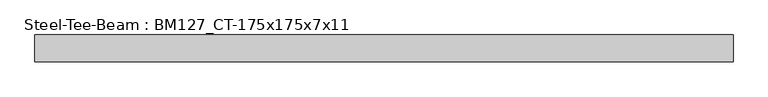
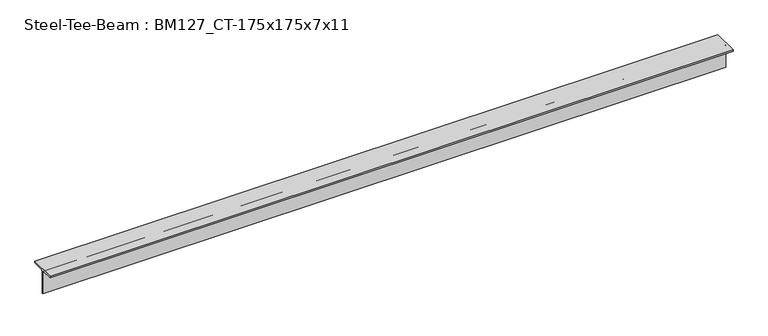
"""IFC4 building model written with IfcOpenShell, lengths in millimetres: beam geometry, Steel-Tee-Beam : BM127_CT-175x175x7x11."""

from ifc_helpers import new_model, si_unit, point, frame, frame_2d, origin, place, context, project, spatial, polyline, circle_curve, trimmed, segment, composite_curve, outline, extrude, source, transform, mapped, element, save


def steel_tee_beam_bm127_ct_175x175x7x11_46f1a80e(model_context):
    return source(origin(), model_context, "Body", "SweptSolid", [
        extrude(outline(composite_curve([segment(polyline([(-87.5, 87.5), (87.5, 87.5), (87.5, 76.5), (17.5, 76.5)]), True, "CONTINUOUS"), segment(trimmed(circle_curve(frame_2d((17.5, 62.5)), 14.0), [point((17.5, 76.5))], [point((3.5, 62.5))], True, "CARTESIAN"), True, "CONTINUOUS"), segment(polyline([(3.5, 62.5), (3.5, -87.5), (-3.5, -87.5), (-3.5, 62.5)]), True, "CONTINUOUS"), segment(trimmed(circle_curve(frame_2d((-17.5, 62.5)), 14.0), [point((-3.5, 62.5))], [point((-17.5, 76.5))], True, "CARTESIAN"), True, "CONTINUOUS"), segment(polyline([(-17.5, 76.5), (-87.5, 76.5), (-87.5, 87.5)]), True, "CONTINUOUS")], self_intersect=False)), frame((-2197.4530821, 0.0, 0.0), z_axis=(1.0, 0.0, 0.0), x_axis=(0.0, 1.0, 0.0)), (0.0, 0.0, 1.0), 4573.2110535),
    ])


if __name__ == "__main__":
    model = new_model("IFC4")
    model_context = context("Model", 3, world=origin())
    ifc_project = project(units=[si_unit("LENGTHUNIT", "METRE", prefix="MILLI")], contexts=[model_context])
    site = spatial("IfcSite", under=ifc_project)
    building = spatial("IfcBuilding", under=site)
    placement = place(None, origin())
    steel_tee_beam_bm127_ct_175x175x7x11_shape = steel_tee_beam_bm127_ct_175x175x7x11_46f1a80e(model_context)
    element("IfcBeam", 1, ObjectType="Steel-Tee-Beam : BM127_CT-175x175x7x11", at=placement, inside=building, context=model_context, shape_type="MappedRepresentation", body=[
        mapped(steel_tee_beam_bm127_ct_175x175x7x11_shape, transform((0.0, 0.0, 0.0), x_axis=(1.0, 0.0, 0.0), y_axis=(0.0, 1.0, 0.0), z_axis=(0.0, 0.0, 1.0))),
    ])
    save(model, "model.ifc")

# Revit data of these elements
# Type "Steel-Tee-Beam : BM127_CT-175x175x7x11"
#   Surface Area = 0.00 m²/m
#   Section Area = 31.57 cm²
#   Mass per Unit Length = 24.80 kg/m
#   Length [instance default] = 1524 mm
#   bf = 175 mm
#   d = 175 mm
#   k = 25 mm
#   kr = 14 mm
#   tf = 11 mm
#   tw = 7 mm
#   hec_material4 [instance default] = none
#   hec_material3 [instance default] = none
#   hec_material2 [instance default] = none
#   hec_material1 [instance default] = none
#   Structural Material [instance default] = Steel, 45-345
#   Assembly Code = ""
# Element 1 (IfcBeam, "Steel-Tee-Beam : BM127_CT-175x175x7x11")
#   hec_material3 = F01AC000-00002_Building/Shelter Fire Proofing Work_Intumescent Coating Type_1 hr. rating (UL 1709))
#   hec_material2 = S01AA010-00002_Main Steel Structure Fabrication Work_Shelter/Building_Steel Painting/Coating_for Fireproofed Steel Surface, Surface Preparation & Primer Coat
#   hec_material1 = S03AA029-00001_Main Steel Structure Erection Work_Shelter/Building_Light Steel
#   Structural Material = S01AA003-00001_Main Steel Structure Fabrication Work_Shelter/Building_Light Steel - Standard
#   Materials on its faces: "S01AA003-00001_Main Steel Structure Fabrication Work_Shelter/Building_Light Steel - Standard"
# Materials
#   "Steel, 45-345": class "Metal", colour RGB 189 187 185, transparency 0, Description = "Steel 345 MPa", Cost = 0
#   "S01AA003-00001_Main Steel Structure Fabrication Work_Shelter/Building_Light Steel - Standard": class "Metal", colour RGB 120 120 120, transparency 0, Comments = "(30KG/M>Weight)", Description = "Structural steel 50ksi", W00) Work Master Code = "S01AA003-00001", W01) Work Master_Lv1 = "Main Steel Structure Fabrication Work", W02) Work Master_Lv2 = "Shelter/Building", W03) Work Master_Spec.1 = "Light Steel - Standard (30KG/M>Weight)", Cost = 0
#   "F01AC000-00002_Building/Shelter Fire Proofing Work_Intumescent Coating Type_1 hr. rating (UL 1709))": class "Metal", colour RGB 255 128 128, transparency 0, Description = "Paint finished steel", W00) Work Master Code = "F01AC000-00002", W01) Work Master_Lv1 = "Building/Shelter Fire Proofing Work", W02) Work Master_Lv2 = "Intumescent Coating Type", W03) Work Master_Spec.1 = "1 hr. rating (UL 1709)", Cost = 0
#   "S01AA010-00002_Main Steel Structure Fabrication Work_Shelter/Building_Steel Painting/Coating_for Fireproofed Steel Surface, Surface Preparation & Primer Coat": class "Metal", colour RGB 120 120 120, transparency 0, Description = "Paint finished steel", W00) Work Master Code = "SS01AA010-00002", W01) Work Master_Lv1 = "Main Steel Structure Fabrication Work", W02) Work Master_Lv2 = "Shelter/Building", W03) Work Master_Spec.1 = "Steel Painting/Coating", W04) Work Master_Spec.2 = "for Fireproofed Steel Surface, Surface Preparation & Primer Coat", Cost = 0
#   "S03AA029-00001_Main Steel Structure Erection Work_Shelter/Building_Light Steel": class "Metal", colour RGB 120 120 120, transparency 0, Comments = "(30KG/M>Weight)", Description = "Structural steel 50ksi", W00) Work Master Code = "S03AA029-00001", W01) Work Master_Lv1 = "Main Steel Structure Erection Work", W02) Work Master_Lv2 = "Shelter/Building", W03) Work Master_Spec.1 = "Light Steel (30KG/M>Weight)", Cost = 0
